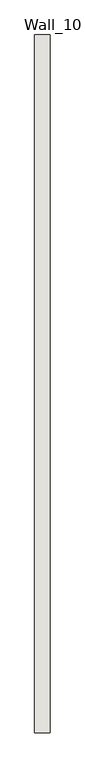
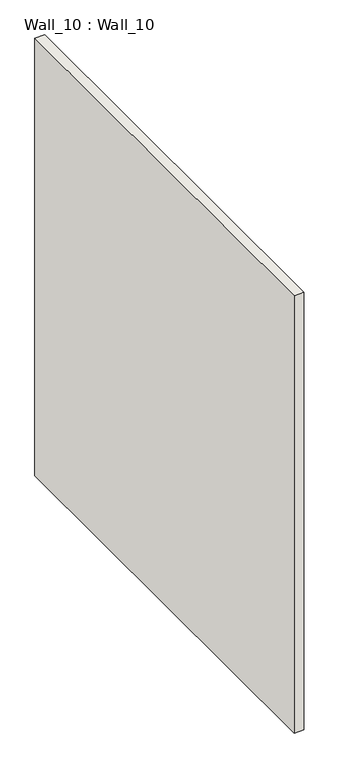
"""IFC4 building model written with IfcOpenShell, lengths in millimetres: wall geometry, Wall_10 : Wall_10."""

from ifc_helpers import new_model, si_unit, origin, origin_with_axes, place, context, project, spatial, polyline, outline, extrude, source, transform, mapped, element, save


def wall_10_wall_10_bc7aa466(model_context):
    return source(origin(), model_context, "Body", "SweptSolid", [
        extrude(outline(polyline([(4480.0, 12090.0), (4480.0, 7530.0), (4380.0, 7530.0), (4380.0, 12090.0), (4480.0, 12090.0)])), origin_with_axes(), (0.0, 0.0, 1.0), 4700.0),
    ])


if __name__ == "__main__":
    model = new_model("IFC4")
    model_context = context("Model", 3, world=origin())
    ifc_project = project(units=[si_unit("LENGTHUNIT", "METRE", prefix="MILLI")], contexts=[model_context])
    site = spatial("IfcSite", under=ifc_project)
    building = spatial("IfcBuilding", under=site)
    placement = place(None, origin())
    wall_10_wall_10_shape = wall_10_wall_10_bc7aa466(model_context)
    element("IfcWall", 1, ObjectType="Wall_10 : Wall_10", at=placement, inside=building, context=model_context, shape_type="MappedRepresentation", body=[
        mapped(wall_10_wall_10_shape, transform((0.0, 0.0, 0.0), x_axis=(1.0, 0.0, 0.0), y_axis=(0.0, 1.0, 0.0), z_axis=(0.0, 0.0, 1.0))),
    ])
    save(model, "model.ifc")

# Revit data of these elements
# Type "Wall_10 : Wall_10"
#   NameOverride = "Wall_10"
# Element 1 (IfcWall, "Wall_10 : Wall_10")
#   Materials on its faces: "IfcSurfaceStyle #33"
# Materials
#   "IfcSurfaceStyle #33": class "Unassigned", colour RGB 214 214 214, transparency 0
